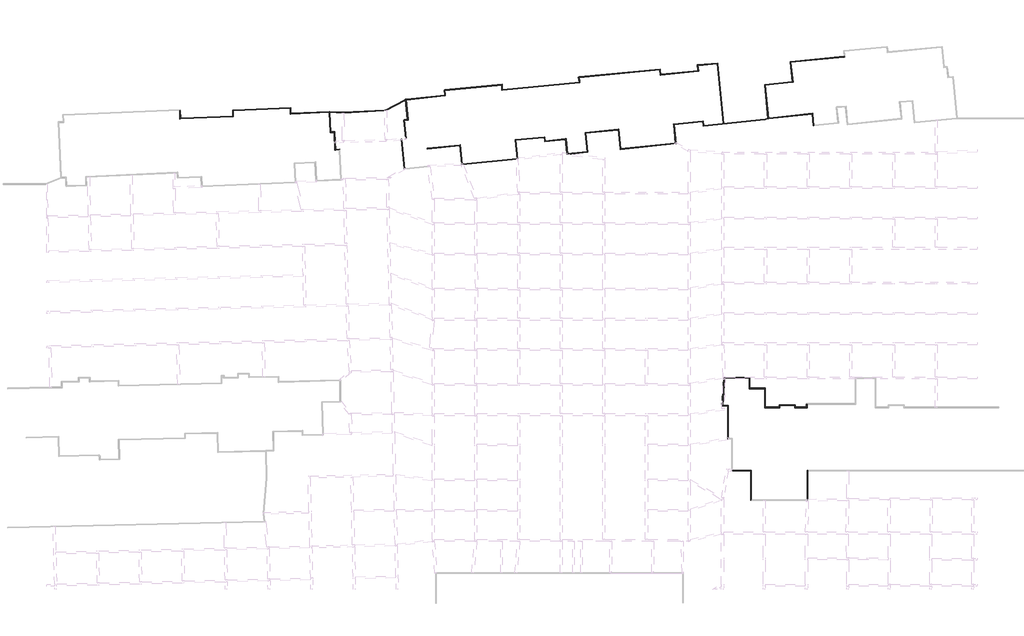
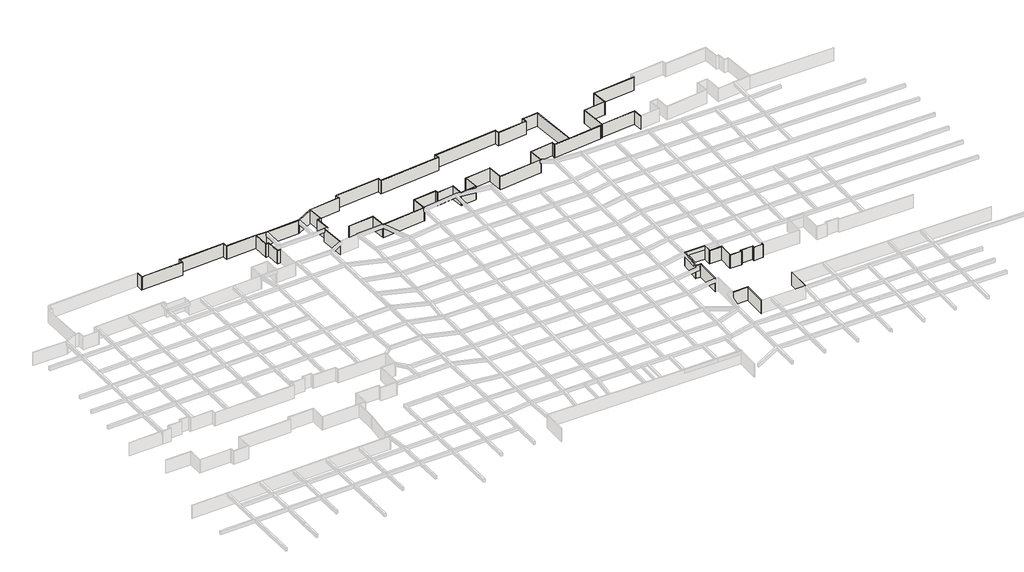
# One storey, part 6 of 20: 69 walls.
"""IFC4 building model written with IfcOpenShell, lengths in millimetres."""

from ifc_helpers import new_model, si_unit, origin, origin_with_axes, place, context, project, spatial, polyline, outline, extrude, faceted_brep, element, save

model = new_model("IFC4")

# Units and contexts
model_context = context("Model", 3, world=origin())
ifc_project = project(units=[si_unit("LENGTHUNIT", "METRE", prefix="MILLI")], contexts=[model_context])

# Site, building, storey
site = spatial("IfcSite", under=ifc_project)
building = spatial("IfcBuilding", under=site)
storey = spatial("IfcBuildingStorey", under=building, Name="户型图", Elevation=0.0)

# Walls
placement = place(None, origin())
element("IfcWall", 1, ObjectType="所有墙体", at=placement, inside=storey, context=model_context, shape_type="Brep", body=[
    faceted_brep([(131729.8124937, 210691.0787424, 0.0), (121574.8609355, 209733.4990588, 0.0), (121574.8609355, 209733.4990588, 3300.0), (131729.8124937, 210691.0787424, 3300.0), (131742.3566275, 210571.7292816, 0.0), (131742.3566275, 210571.7292816, 3300.0), (121706.8819283, 209625.4158865, 3300.0), (121587.4050693, 209614.1495981, 3300.0), (121587.4050693, 209614.1495981, 0.0), (121706.8819283, 209625.4158865, 0.0)], [[[0, 1, 2, 3]], [[4, 5, 6, 7, 8, 9]], [[1, 0, 4, 9, 8]], [[3, 2, 7, 6, 5]], [[0, 3, 5, 4]], [[2, 1, 8, 7]]]),
])
element("IfcWall", 2, ObjectType="所有墙体", at=placement, inside=storey, context=model_context, shape_type="Brep", body=[
    faceted_brep([(121587.4050693, 209614.1495981, 0.0), (121972.1365708, 205953.6738762, 0.0), (121984.6799864, 205834.3312487, 0.0), (121984.6799864, 205834.3312487, 3300.0), (121972.1365708, 205953.6738762, 3300.0), (121587.4050693, 209614.1495981, 3300.0), (121706.8819283, 209625.4158865, 0.0), (121706.8819283, 209625.4158865, 3300.0), (122104.0226138, 205846.8746643, 3300.0), (122104.0226138, 205846.8746643, 0.0)], [[[0, 1, 2, 3, 4, 5]], [[6, 7, 8, 9]], [[2, 1, 0, 6, 9]], [[5, 4, 3, 8, 7]], [[0, 5, 7, 6]], [[3, 2, 9, 8]]]),
])
element("IfcWall", 3, ObjectType="所有墙体", at=placement, inside=storey, context=model_context, shape_type="Brep", body=[
    faceted_brep([(121972.1365708, 205953.6738762, 0.0), (116800.5870466, 205410.1221183, 0.0), (116800.5870466, 205410.1221183, 3300.0), (121972.1365708, 205953.6738762, 3300.0), (121984.6799864, 205834.3312487, 0.0), (121984.6799864, 205834.3312487, 3300.0), (116931.2027957, 205303.1893932, 3300.0), (116811.853335, 205290.6452594, 3300.0), (116811.853335, 205290.6452594, 0.0), (116931.2027957, 205303.1893932, 0.0)], [[[0, 1, 2, 3]], [[4, 5, 6, 7, 8, 9]], [[1, 0, 4, 9, 8]], [[3, 2, 7, 6, 5]], [[0, 3, 5, 4]], [[2, 1, 8, 7]]]),
])
element("IfcWall", 4, ObjectType="所有墙体", at=placement, inside=storey, context=model_context, shape_type="Brep", body=[
    faceted_brep([(116811.853335, 205290.6452594, 0.0), (117393.2536778, 199125.0045105, 0.0), (117404.8959314, 199001.5406116, 0.0), (117404.8959314, 199001.5406116, 3300.0), (117393.2536778, 199125.0045105, 3300.0), (116811.853335, 205290.6452594, 3300.0), (116931.2027957, 205303.1893932, 0.0), (116931.2027957, 205303.1893932, 3300.0), (117521.4287148, 199043.9550761, 3300.0), (117521.4287148, 199043.9550761, 0.0)], [[[0, 1, 2, 3, 4, 5]], [[6, 7, 8, 9]], [[2, 1, 0, 6, 9]], [[5, 4, 3, 8, 7]], [[0, 5, 7, 6]], [[3, 2, 9, 8]]]),
])
element("IfcWall", 5, ObjectType="所有墙体", at=placement, inside=storey, context=model_context, shape_type="SweptSolid", body=[
    extrude(outline(polyline([(116894.9852677, 198943.6496406), (117393.2536778, 199125.0045105), (117404.8959314, 199001.5406116), (116922.1821154, 198825.8471509), (116894.9852677, 198943.6496406)])), origin_with_axes(), (0.0, 0.0, 1.0), 3300.0),
])
element("IfcWall", 6, ObjectType="所有墙体", at=placement, inside=storey, context=model_context, shape_type="Brep", body=[
    faceted_brep([(116894.9852677, 198943.6496406, 0.0), (109153.4306479, 198129.9794625, 0.0), (109034.0880204, 198117.4360469, 0.0), (105355.2231692, 197730.7717701, 0.0), (105235.8805418, 197718.2283545, 0.0), (105235.8805418, 197718.2283545, 3300.0), (105355.2231692, 197730.7717701, 3300.0), (109034.0880204, 198117.4360469, 3300.0), (109153.4306479, 198129.9794625, 3300.0), (116894.9852677, 198943.6496406, 3300.0), (116922.1821154, 198825.8471509, 0.0), (116922.1821154, 198825.8471509, 3300.0), (105248.4239574, 197598.885727, 3300.0), (105248.4239574, 197598.885727, 0.0)], [[[0, 1, 2, 3, 4, 5, 6, 7, 8, 9]], [[10, 11, 12, 13]], [[4, 3, 2, 1, 0, 10, 13]], [[9, 8, 7, 6, 5, 12, 11]], [[0, 9, 11, 10]], [[5, 4, 13, 12]]]),
])
element("IfcWall", 7, ObjectType="所有墙体", at=placement, inside=storey, context=model_context, shape_type="Brep", body=[
    faceted_brep([(105355.2231692, 197730.7717701, 0.0), (105266.7980678, 198572.0804116, 0.0), (105266.7980678, 198572.0804116, 3300.0), (105355.2231692, 197730.7717701, 3300.0), (105235.8805418, 197718.2283545, 0.0), (105235.8805418, 197718.2283545, 3300.0), (105159.998856, 198440.1943685, 3300.0), (105147.4554404, 198559.536996, 3300.0), (105147.4554404, 198559.536996, 0.0), (105159.998856, 198440.1943685, 0.0)], [[[0, 1, 2, 3]], [[4, 5, 6, 7, 8, 9]], [[1, 0, 4, 9, 8]], [[3, 2, 7, 6, 5]], [[0, 3, 5, 4]], [[2, 1, 8, 7]]]),
])
element("IfcWall", 8, ObjectType="所有墙体", at=placement, inside=storey, context=model_context, shape_type="Brep", body=[
    faceted_brep([(105147.4554404, 198559.536996, 0.0), (99683.6940432, 197985.2725327, 0.0), (99683.6940432, 197985.2725327, 3300.0), (105147.4554404, 198559.536996, 3300.0), (105159.998856, 198440.1943685, 0.0), (105159.998856, 198440.1943685, 3300.0), (99815.5800862, 197878.4733208, 3300.0), (99696.2374587, 197865.9299052, 3300.0), (99696.2374587, 197865.9299052, 0.0), (99815.5800862, 197878.4733208, 0.0)], [[[0, 1, 2, 3]], [[4, 5, 6, 7, 8, 9]], [[1, 0, 4, 9, 8]], [[3, 2, 7, 6, 5]], [[0, 3, 5, 4]], [[2, 1, 8, 7]]]),
])
element("IfcWall", 9, ObjectType="所有墙体", at=placement, inside=storey, context=model_context, shape_type="Brep", body=[
    faceted_brep([(99696.2374587, 197865.9299052, 0.0), (100056.1217007, 194441.8600656, 0.0), (100068.6651163, 194322.5174382, 0.0), (100068.6651163, 194322.5174382, 3300.0), (100056.1217007, 194441.8600656, 3300.0), (99696.2374587, 197865.9299052, 3300.0), (99815.5800862, 197878.4733208, 0.0), (99815.5800862, 197878.4733208, 3300.0), (100188.0077438, 194335.0608538, 3300.0), (100188.0077438, 194335.0608538, 0.0)], [[[0, 1, 2, 3, 4, 5]], [[6, 7, 8, 9]], [[2, 1, 0, 6, 9]], [[5, 4, 3, 8, 7]], [[0, 5, 7, 6]], [[3, 2, 9, 8]]]),
])
element("IfcWall", 10, ObjectType="所有墙体", at=placement, inside=storey, context=model_context, shape_type="Brep", body=[
    faceted_brep([(100056.1217007, 194441.8600656, 0.0), (89808.126809, 193364.7523995, 0.0), (89688.7841816, 193352.2089839, 0.0), (89688.7841816, 193352.2089839, 3300.0), (89808.126809, 193364.7523995, 3300.0), (100056.1217007, 194441.8600656, 3300.0), (100068.6651163, 194322.5174382, 0.0), (100068.6651163, 194322.5174382, 3300.0), (89701.3275972, 193232.8663565, 3300.0), (89701.3275972, 193232.8663565, 0.0)], [[[0, 1, 2, 3, 4, 5]], [[6, 7, 8, 9]], [[2, 1, 0, 6, 9]], [[5, 4, 3, 8, 7]], [[0, 5, 7, 6]], [[3, 2, 9, 8]]]),
])
element("IfcWall", 11, ObjectType="所有墙体", at=placement, inside=storey, context=model_context, shape_type="Brep", body=[
    faceted_brep([(89808.126809, 193364.7523995, 0.0), (89421.371495, 197044.4834124, 0.0), (89421.371495, 197044.4834124, 3300.0), (89808.126809, 193364.7523995, 3300.0), (89688.7841816, 193352.2089839, 0.0), (89688.7841816, 193352.2089839, 3300.0), (89314.5722831, 196912.5973693, 3300.0), (89302.0288675, 197031.9399968, 3300.0), (89302.0288675, 197031.9399968, 0.0), (89314.5722831, 196912.5973693, 0.0)], [[[0, 1, 2, 3]], [[4, 5, 6, 7, 8, 9]], [[1, 0, 4, 9, 8]], [[3, 2, 7, 6, 5]], [[0, 3, 5, 4]], [[2, 1, 8, 7]]]),
])
element("IfcWall", 12, ObjectType="所有墙体", at=placement, inside=storey, context=model_context, shape_type="Brep", body=[
    faceted_brep([(89302.0288675, 197031.9399968, 0.0), (83160.2882507, 196386.4170461, 0.0), (83160.2882507, 196386.4170461, 3300.0), (89302.0288675, 197031.9399968, 3300.0), (89314.5722831, 196912.5973693, 0.0), (89314.5722831, 196912.5973693, 3300.0), (83292.1742938, 196279.6178342, 3300.0), (83172.8316663, 196267.0744186, 3300.0), (83172.8316663, 196267.0744186, 0.0), (83292.1742938, 196279.6178342, 0.0)], [[[0, 1, 2, 3]], [[4, 5, 6, 7, 8, 9]], [[1, 0, 4, 9, 8]], [[3, 2, 7, 6, 5]], [[0, 3, 5, 4]], [[2, 1, 8, 7]]]),
])
element("IfcWall", 13, ObjectType="所有墙体", at=placement, inside=storey, context=model_context, shape_type="Brep", body=[
    faceted_brep([(83172.8316663, 196267.0744186, 0.0), (83535.1177075, 192820.1529861, 0.0), (83547.6611231, 192700.8103587, 0.0), (83547.6611231, 192700.8103587, 3300.0), (83535.1177075, 192820.1529861, 3300.0), (83172.8316663, 196267.0744186, 3300.0), (83292.1742938, 196279.6178342, 0.0), (83292.1742938, 196279.6178342, 3300.0), (83667.0037505, 192713.3537743, 3300.0), (83667.0037505, 192713.3537743, 0.0)], [[[0, 1, 2, 3, 4, 5]], [[6, 7, 8, 9]], [[2, 1, 0, 6, 9]], [[5, 4, 3, 8, 7]], [[0, 5, 7, 6]], [[3, 2, 9, 8]]]),
])
element("IfcWall", 14, ObjectType="所有墙体", at=placement, inside=storey, context=model_context, shape_type="Brep", body=[
    faceted_brep([(83535.1177075, 192820.1529861, 0.0), (79847.9790856, 192432.6191009, 0.0), (79728.6364581, 192420.0756853, 0.0), (79728.6364581, 192420.0756853, 3300.0), (79847.9790856, 192432.6191009, 3300.0), (80284.9846417, 192478.5502357, 3300.0), (83535.1177075, 192820.1529861, 3300.0), (83547.6611231, 192700.8103587, 0.0), (83547.6611231, 192700.8103587, 3300.0), (80814.4577688, 192413.5391103, 3300.0), (79741.1798737, 192300.7330579, 3300.0), (79741.1798737, 192300.7330579, 2500.0), (79741.1798737, 192300.7330579, 0.0)], [[[0, 1, 2, 3, 4, 5, 6]], [[7, 8, 9, 10, 11, 12]], [[2, 1, 0, 7, 12]], [[6, 5, 4, 3, 10, 9, 8]], [[0, 6, 8, 7]], [[3, 2, 12, 11, 10]]]),
])
element("IfcWall", 15, ObjectType="所有墙体", at=placement, inside=storey, context=model_context, shape_type="Brep", body=[
    faceted_brep([(79847.9790856, 192432.6191009, 0.0), (79552.5957881, 195243.0034464, 0.0), (79552.5957881, 195243.0034464, 3300.0), (79837.3750476, 192533.5097832, 3300.0), (79847.9790856, 192432.6191009, 3300.0), (79847.9790856, 192432.6191009, 2500.0), (79728.6364581, 192420.0756853, 0.0), (79728.6364581, 192420.0756853, 3300.0), (79715.1365445, 192548.5187841, 3300.0), (79445.7965763, 195111.1174033, 3300.0), (79433.2531607, 195230.4600308, 3300.0), (79433.2531607, 195230.4600308, 0.0), (79445.7965763, 195111.1174033, 0.0)], [[[0, 1, 2, 3, 4, 5]], [[6, 7, 8, 9, 10, 11, 12]], [[1, 0, 6, 12, 11]], [[4, 3, 2, 10, 9, 8, 7]], [[0, 5, 4, 7, 6]], [[2, 1, 11, 10]]]),
])
element("IfcWall", 16, ObjectType="所有墙体", at=placement, inside=storey, context=model_context, shape_type="Brep", body=[
    faceted_brep([(79433.2531607, 195230.4600308, 0.0), (75644.1175717, 194832.2058324, 0.0), (75524.7749443, 194819.6624168, 0.0), (75524.7749443, 194819.6624168, 3300.0), (75644.1175717, 194832.2058324, 3300.0), (79433.2531607, 195230.4600308, 3300.0), (79445.7965763, 195111.1174033, 0.0), (79445.7965763, 195111.1174033, 3300.0), (75537.3183598, 194700.3197894, 3300.0), (75537.3183598, 194700.3197894, 0.0)], [[[0, 1, 2, 3, 4, 5]], [[6, 7, 8, 9]], [[2, 1, 0, 6, 9]], [[5, 4, 3, 8, 7]], [[0, 5, 7, 6]], [[3, 2, 9, 8]]]),
])
element("IfcWall", 17, ObjectType="所有墙体", at=placement, inside=storey, context=model_context, shape_type="Brep", body=[
    faceted_brep([(75644.1175717, 194832.2058324, 0.0), (75564.7799301, 195587.0530699, 0.0), (75564.7799301, 195587.0530699, 3300.0), (75644.1175717, 194832.2058324, 3300.0), (75524.7749443, 194819.6624168, 0.0), (75524.7749443, 194819.6624168, 3300.0), (75457.7636828, 195457.2319809, 3300.0), (75445.2183565, 195576.5927876, 3300.0), (75445.2183565, 195576.5927876, 0.0), (75457.7636828, 195457.2319809, 0.0)], [[[0, 1, 2, 3]], [[4, 5, 6, 7, 8, 9]], [[1, 0, 4, 9, 8]], [[3, 2, 7, 6, 5]], [[0, 3, 5, 4]], [[2, 1, 8, 7]]]),
])
element("IfcWall", 18, ObjectType="所有墙体", at=placement, inside=storey, context=model_context, shape_type="Brep", body=[
    faceted_brep([(75445.2183565, 195576.5927876, 0.0), (69986.0714109, 195098.9793173, 0.0), (69986.0714109, 195098.9793173, 3300.0), (75445.2183565, 195576.5927876, 3300.0), (75457.7636828, 195457.2319809, 0.0), (75457.7636828, 195457.2319809, 3300.0), (70118.1783108, 194990.0787929, 3300.0), (69998.6167372, 194979.6185106, 3300.0), (69998.6167372, 194979.6185106, 0.0), (70118.1783108, 194990.0787929, 0.0)], [[[0, 1, 2, 3]], [[4, 5, 6, 7, 8, 9]], [[1, 0, 4, 9, 8]], [[3, 2, 7, 6, 5]], [[0, 3, 5, 4]], [[2, 1, 8, 7]]]),
])
element("IfcWall", 19, ObjectType="所有墙体", at=placement, inside=storey, context=model_context, shape_type="Brep", body=[
    faceted_brep([(69998.6167372, 194979.6185106, 0.0), (70362.4316658, 191518.1506866, 0.0), (70374.9755195, 191398.8038903, 0.0), (70374.9755195, 191398.8038903, 3300.0), (70362.4316658, 191518.1506866, 3300.0), (69998.6167372, 194979.6185106, 3300.0), (70118.1783108, 194990.0787929, 0.0), (70118.1783108, 194990.0787929, 3300.0), (70494.4229915, 191410.349777, 3300.0), (70494.4229915, 191410.349777, 0.0)], [[[0, 1, 2, 3, 4, 5]], [[6, 7, 8, 9]], [[2, 1, 0, 6, 9]], [[5, 4, 3, 8, 7]], [[0, 5, 7, 6]], [[3, 2, 9, 8]]]),
])
element("IfcWall", 20, ObjectType="所有墙体", at=placement, inside=storey, context=model_context, shape_type="Brep", body=[
    faceted_brep([(70362.4316658, 191518.1506866, 0.0), (60092.4518091, 190525.4463415, 0.0), (59973.0043371, 190513.9004548, 0.0), (59973.0043371, 190513.9004548, 3300.0), (60092.4518091, 190525.4463415, 3300.0), (70362.4316658, 191518.1506866, 3300.0), (70374.9755195, 191398.8038903, 0.0), (70374.9755195, 191398.8038903, 3300.0), (59985.5481909, 190394.5536585, 3300.0), (59985.5481909, 190394.5536585, 0.0)], [[[0, 1, 2, 3, 4, 5]], [[6, 7, 8, 9]], [[2, 1, 0, 6, 9]], [[5, 4, 3, 8, 7]], [[0, 5, 7, 6]], [[3, 2, 9, 8]]]),
])
element("IfcWall", 21, ObjectType="所有墙体", at=placement, inside=storey, context=model_context, shape_type="Brep", body=[
    faceted_brep([(60092.4518091, 190525.4463415, 0.0), (59716.0971382, 194106.2218448, 0.0), (59716.0971382, 194106.2218448, 3300.0), (60092.4518091, 190525.4463415, 3300.0), (59973.0043371, 190513.9004548, 0.0), (59973.0043371, 190513.9004548, 3300.0), (59609.2979263, 193974.3358018, 3300.0), (59596.7545107, 194093.6784293, 3300.0), (59596.7545107, 194093.6784293, 0.0), (59609.2979263, 193974.3358018, 0.0)], [[[0, 1, 2, 3]], [[4, 5, 6, 7, 8, 9]], [[1, 0, 4, 9, 8]], [[3, 2, 7, 6, 5]], [[0, 3, 5, 4]], [[2, 1, 8, 7]]]),
])
element("IfcWall", 22, ObjectType="所有墙体", at=placement, inside=storey, context=model_context, shape_type="SweptSolid", body=[
    extrude(outline(polyline([(53516.2635964, 193454.5930817), (59596.7545107, 194093.6784293), (59609.2979263, 193974.3358018), (53528.8070119, 193335.2504542), (53516.2635964, 193454.5930817)])), origin_with_axes(), (0.0, 0.0, 1.0), 3300.0),
])
element("IfcWall", 23, ObjectType="所有墙体", at=placement, inside=storey, context=model_context, shape_type="Brep", body=[
    faceted_brep([(48667.2783502, 195165.2272583, 0.0), (49211.8887729, 189530.9836906, 0.0), (49211.8887729, 189530.9836906, 3300.0), (48684.0697224, 194991.5128437, 3300.0), (48667.2783502, 195165.2272583, 3300.0), (48667.2783502, 195165.2272583, 2500.0), (48786.7216498, 195176.7727417, 0.0), (48786.7216498, 195176.7727417, 2500.0), (48786.7216498, 195176.7727417, 3300.0), (48803.4165187, 195004.0566974, 3300.0), (49319.6896824, 189662.9750163, 3300.0), (49331.2355692, 189543.5275444, 3300.0), (49331.2355692, 189543.5275444, 0.0), (49319.6896824, 189662.9750163, 0.0)], [[[0, 1, 2, 3, 4, 5]], [[6, 7, 8, 9, 10, 11, 12, 13]], [[1, 0, 6, 13, 12]], [[4, 3, 2, 11, 10, 9, 8]], [[0, 5, 4, 8, 7, 6]], [[2, 1, 12, 11]]]),
])
element("IfcWall", 24, ObjectType="所有墙体", at=placement, inside=storey, context=model_context, shape_type="Brep", body=[
    faceted_brep([(49582.7742245, 195254.2236424, 0.0), (49223.1963109, 198675.3789625, 0.0), (49210.6528953, 198794.7215899, 0.0), (49210.6528953, 198794.7215899, 3300.0), (49223.1963109, 198675.3789625, 3300.0), (49582.7742245, 195254.2236424, 3300.0), (49463.4315971, 195241.6802268, 0.0), (49463.4315971, 195241.6802268, 3300.0), (49091.3102679, 198782.1781744, 3300.0), (49091.3102679, 198782.1781744, 0.0)], [[[0, 1, 2, 3, 4, 5]], [[6, 7, 8, 9]], [[2, 1, 0, 6, 9]], [[5, 4, 3, 8, 7]], [[0, 5, 7, 6]], [[3, 2, 9, 8]]]),
])
element("IfcWall", 25, ObjectType="所有墙体", at=placement, inside=storey, context=model_context, shape_type="Brep", body=[
    faceted_brep([(49223.1963109, 198675.3789625, 0.0), (49941.1246624, 198750.8362729, 0.0), (49941.1246624, 198750.8362729, 3300.0), (49223.1963109, 198675.3789625, 3300.0), (49210.6528953, 198794.7215899, 0.0), (49210.6528953, 198794.7215899, 3300.0), (49810.2319794, 198857.7398911, 3300.0), (49929.5787757, 198870.2837448, 3300.0), (49929.5787757, 198870.2837448, 0.0), (49810.2319794, 198857.7398911, 0.0)], [[[0, 1, 2, 3]], [[4, 5, 6, 7, 8, 9]], [[1, 0, 4, 9, 8]], [[3, 2, 7, 6, 5]], [[0, 3, 5, 4]], [[2, 1, 8, 7]]]),
])
element("IfcWall", 26, ObjectType="所有墙体", at=placement, inside=storey, context=model_context, shape_type="Brep", body=[
    faceted_brep([(49929.5787757, 198870.2837448, 0.0), (49575.5176865, 202533.2074259, 0.0), (49563.9717998, 202652.6548978, 0.0), (49563.9717998, 202652.6548978, 3300.0), (49575.5176865, 202533.2074259, 3300.0), (49929.5787757, 198870.2837448, 3300.0), (49810.2319794, 198857.7398911, 0.0), (49810.2319794, 198857.7398911, 3300.0), (49458.9857705, 202491.5423501, 3300.0), (49446.4909346, 202620.8071341, 3300.0), (49444.6250035, 202640.1110441, 3300.0), (49444.6250035, 202640.1110441, 0.0), (49446.4909346, 202620.8071341, 0.0), (49458.9857705, 202491.5423501, 0.0)], [[[0, 1, 2, 3, 4, 5]], [[6, 7, 8, 9, 10, 11, 12, 13]], [[2, 1, 0, 6, 13, 12, 11]], [[5, 4, 3, 10, 9, 8, 7]], [[0, 5, 7, 6]], [[3, 2, 11, 10]]]),
])
element("IfcWall", 27, ObjectType="所有墙体", at=placement, inside=storey, context=model_context, shape_type="Brep", body=[
    faceted_brep([(49575.5176865, 202533.2074259, 0.0), (56935.4763922, 203306.7702572, 0.0), (56935.4763922, 203306.7702572, 3300.0), (49575.5176865, 202533.2074259, 3300.0), (49563.9717998, 202652.6548978, 0.0), (49563.9717998, 202652.6548978, 3300.0), (56803.5903492, 203413.5694691, 3300.0), (56922.9329766, 203426.1128847, 3300.0), (56922.9329766, 203426.1128847, 0.0), (56803.5903492, 203413.5694691, 0.0)], [[[0, 1, 2, 3]], [[4, 5, 6, 7, 8, 9]], [[1, 0, 4, 9, 8]], [[3, 2, 7, 6, 5]], [[0, 3, 5, 4]], [[2, 1, 8, 7]]]),
])
element("IfcWall", 28, ObjectType="所有墙体", at=placement, inside=storey, context=model_context, shape_type="Brep", body=[
    faceted_brep([(56922.9329766, 203426.1128847, 0.0), (56831.5181439, 204295.8669196, 0.0), (56818.9742902, 204415.2137159, 0.0), (56818.9742902, 204415.2137159, 3300.0), (56831.5181439, 204295.8669196, 3300.0), (56922.9329766, 203426.1128847, 3300.0), (56803.5903492, 203413.5694691, 0.0), (56803.5903492, 203413.5694691, 3300.0), (56699.5268182, 204403.6678292, 3300.0), (56699.5268182, 204403.6678292, 0.0)], [[[0, 1, 2, 3, 4, 5]], [[6, 7, 8, 9]], [[2, 1, 0, 6, 9]], [[5, 4, 3, 8, 7]], [[0, 5, 7, 6]], [[3, 2, 9, 8]]]),
])
element("IfcWall", 29, ObjectType="所有墙体", at=placement, inside=storey, context=model_context, shape_type="Brep", body=[
    faceted_brep([(56831.5181439, 204295.8669196, 0.0), (67455.4194423, 205322.7815901, 0.0), (67575.4194423, 205334.3808846, 0.0), (67575.4194423, 205334.3808846, 3300.0), (67455.4194423, 205322.7815901, 3300.0), (56831.5181439, 204295.8669196, 3300.0), (56818.9742902, 204415.2137159, 0.0), (56818.9742902, 204415.2137159, 3300.0), (67575.4194423, 205454.9401797, 3300.0), (67575.4194423, 205454.9401797, 0.0)], [[[0, 1, 2, 3, 4, 5]], [[6, 7, 8, 9]], [[2, 1, 0, 6, 9]], [[5, 4, 3, 8, 7]], [[0, 5, 7, 6]], [[3, 2, 9, 8]]]),
])
element("IfcWall", 30, ObjectType="所有墙体", at=placement, inside=storey, context=model_context, shape_type="Brep", body=[
    faceted_brep([(67455.4194423, 205322.7815901, 0.0), (67455.4194423, 204322.7815901, 0.0), (67455.4194423, 204322.7815901, 3300.0), (67455.4194423, 205322.7815901, 3300.0), (67575.4194423, 205334.3808846, 0.0), (67575.4194423, 205334.3808846, 3300.0), (67575.4194423, 204454.9401797, 3300.0), (67575.4194423, 204334.3808846, 3300.0), (67575.4194423, 204334.3808846, 0.0), (67575.4194423, 204454.9401797, 0.0)], [[[0, 1, 2, 3]], [[4, 5, 6, 7, 8, 9]], [[1, 0, 4, 9, 8]], [[3, 2, 7, 6, 5]], [[0, 3, 5, 4]], [[2, 1, 8, 7]]]),
])
element("IfcWall", 31, ObjectType="所有墙体", at=placement, inside=storey, context=model_context, shape_type="Brep", body=[
    faceted_brep([(67575.4194423, 204334.3808846, 0.0), (82113.181948, 205739.6124633, 0.0), (82113.181948, 205739.6124633, 3300.0), (67575.4194423, 204334.3808846, 3300.0), (67575.4194423, 204454.9401797, 0.0), (67575.4194423, 204454.9401797, 3300.0), (81982.193165, 205847.5102794, 3300.0), (82101.6364646, 205859.0557628, 3300.0), (82101.6364646, 205859.0557628, 0.0), (81982.193165, 205847.5102794, 0.0)], [[[0, 1, 2, 3]], [[4, 5, 6, 7, 8, 9]], [[1, 0, 4, 9, 8]], [[3, 2, 7, 6, 5]], [[0, 3, 5, 4]], [[2, 1, 8, 7]]]),
])
element("IfcWall", 32, ObjectType="所有墙体", at=placement, inside=storey, context=model_context, shape_type="Brep", body=[
    faceted_brep([(81886.4271484, 206838.2534608, 0.0), (81982.193165, 205847.5102794, 0.0), (81982.193165, 205847.5102794, 3300.0), (81886.4271484, 206838.2534608, 3300.0), (82005.870448, 206849.7989442, 0.0), (82005.870448, 206849.7989442, 3300.0), (82017.4159314, 206730.3556446, 3300.0), (82101.6364646, 205859.0557628, 3300.0), (82101.6364646, 205859.0557628, 0.0), (82017.4159314, 206730.3556446, 0.0)], [[[0, 1, 2, 3]], [[4, 5, 6, 7, 8, 9]], [[1, 0, 4, 9, 8]], [[3, 2, 7, 6, 5]], [[2, 1, 8, 7]], [[0, 3, 5, 4]]]),
])
element("IfcWall", 33, ObjectType="所有墙体", at=placement, inside=storey, context=model_context, shape_type="Brep", body=[
    faceted_brep([(82017.4159314, 206730.3556446, 0.0), (97124.0566493, 208190.5754395, 0.0), (97243.4999488, 208202.120923, 0.0), (97243.4999488, 208202.120923, 3300.0), (97124.0566493, 208190.5754395, 3300.0), (82017.4159314, 206730.3556446, 3300.0), (82005.870448, 206849.7989442, 0.0), (82005.870448, 206849.7989442, 3300.0), (97231.9544654, 208321.5642225, 3300.0), (97231.9544654, 208321.5642225, 0.0)], [[[0, 1, 2, 3, 4, 5]], [[6, 7, 8, 9]], [[2, 1, 0, 6, 9]], [[5, 4, 3, 8, 7]], [[0, 5, 7, 6]], [[3, 2, 9, 8]]]),
])
element("IfcWall", 34, ObjectType="所有墙体", at=placement, inside=storey, context=model_context, shape_type="Brep", body=[
    faceted_brep([(97124.0566493, 208190.5754395, 0.0), (97219.1952312, 207206.3233554, 0.0), (97219.1952312, 207206.3233554, 3300.0), (97124.0566493, 208190.5754395, 3300.0), (97243.4999488, 208202.120923, 0.0), (97243.4999488, 208202.120923, 3300.0), (97327.0930474, 207337.3121384, 3300.0), (97338.6385308, 207217.8688388, 3300.0), (97338.6385308, 207217.8688388, 0.0), (97327.0930474, 207337.3121384, 0.0)], [[[0, 1, 2, 3]], [[4, 5, 6, 7, 8, 9]], [[1, 0, 4, 9, 8]], [[3, 2, 7, 6, 5]], [[0, 3, 5, 4]], [[2, 1, 8, 7]]]),
])
element("IfcWall", 35, ObjectType="所有墙体", at=placement, inside=storey, context=model_context, shape_type="Brep", body=[
    faceted_brep([(97338.6385308, 207217.8688388, 0.0), (104406.2016933, 207901.0250629, 0.0), (104406.2016933, 207901.0250629, 3300.0), (97338.6385308, 207217.8688388, 3300.0), (97327.0930474, 207337.3121384, 0.0), (97327.0930474, 207337.3121384, 3300.0), (104274.2103676, 208008.8259724, 3300.0), (104393.6578396, 208020.3718592, 3300.0), (104393.6578396, 208020.3718592, 0.0), (104274.2103676, 208008.8259724, 0.0)], [[[0, 1, 2, 3]], [[4, 5, 6, 7, 8, 9]], [[1, 0, 4, 9, 8]], [[3, 2, 7, 6, 5]], [[0, 3, 5, 4]], [[2, 1, 8, 7]]]),
])
element("IfcWall", 36, ObjectType="所有墙体", at=placement, inside=storey, context=model_context, shape_type="Brep", body=[
    faceted_brep([(104393.6578396, 208020.3718592, 0.0), (104291.2203837, 208994.9991478, 0.0), (104278.67653, 209114.3459441, 0.0), (104278.67653, 209114.3459441, 3300.0), (104291.2203837, 208994.9991478, 3300.0), (104393.6578396, 208020.3718592, 3300.0), (104274.2103676, 208008.8259724, 0.0), (104274.2103676, 208008.8259724, 3300.0), (104159.229058, 209102.8000573, 3300.0), (104159.229058, 209102.8000573, 0.0)], [[[0, 1, 2, 3, 4, 5]], [[6, 7, 8, 9]], [[2, 1, 0, 6, 9]], [[5, 4, 3, 8, 7]], [[0, 5, 7, 6]], [[3, 2, 9, 8]]]),
])
element("IfcWall", 37, ObjectType="所有墙体", at=placement, inside=storey, context=model_context, shape_type="Brep", body=[
    faceted_brep([(104291.2203837, 208994.9991478, 0.0), (107854.6079818, 209339.4390007, 0.0), (107974.0554538, 209350.9848875, 0.0), (107974.0554538, 209350.9848875, 3300.0), (107854.6079818, 209339.4390007, 3300.0), (104291.2203837, 208994.9991478, 3300.0), (104278.67653, 209114.3459441, 0.0), (104278.67653, 209114.3459441, 3300.0), (107961.5116, 209470.3316838, 3300.0), (107961.5116, 209470.3316838, 0.0)], [[[0, 1, 2, 3, 4, 5]], [[6, 7, 8, 9]], [[2, 1, 0, 6, 9]], [[5, 4, 3, 8, 7]], [[0, 5, 7, 6]], [[3, 2, 9, 8]]]),
])
element("IfcWall", 38, ObjectType="所有墙体", at=placement, inside=storey, context=model_context, shape_type="SweptSolid", body=[
    extrude(outline(polyline([(109034.0880204, 198117.4360469), (107854.6079818, 209339.4390007), (107974.0554538, 209350.9848875), (109153.4306479, 198129.9794625), (109034.0880204, 198117.4360469)])), origin_with_axes(), (0.0, 0.0, 1.0), 3300.0),
])
element("IfcWall", 39, ObjectType="所有墙体", at=placement, inside=storey, context=model_context, shape_type="Brep", body=[
    faceted_brep([(49446.4909346, 202620.8071341, 0.0), (45696.9730881, 200627.153131, 0.0), (45446.265249, 200493.8494083, 0.0), (45446.265249, 200493.8494083, 3300.0), (45696.9730881, 200627.153131, 3300.0), (49446.4909346, 202620.8071341, 3300.0), (49458.9857705, 202491.5423501, 0.0), (49458.9857705, 202491.5423501, 3300.0), (45729.8203033, 200508.709899, 3300.0), (45729.8203033, 200508.709899, 0.0)], [[[0, 1, 2, 3, 4, 5]], [[6, 7, 8, 9]], [[2, 1, 0, 6, 9]], [[5, 4, 3, 8, 7]], [[0, 5, 7, 6]], [[3, 2, 9, 8]]]),
])
element("IfcWall", 40, ObjectType="所有墙体", at=placement, inside=storey, context=model_context, shape_type="SweptSolid", body=[
    extrude(outline(polyline([(37724.3604177, 200209.3262058), (45696.9730881, 200627.153131), (45446.265249, 200493.8494083), (37724.3604177, 200089.1615243), (37724.3604177, 200209.3262058)])), origin_with_axes(), (0.0, 0.0, 1.0), 3300.0),
])
element("IfcWall", 41, ObjectType="所有墙体", at=placement, inside=storey, context=model_context, shape_type="Brep", body=[
    faceted_brep([(37724.3604177, 200209.3262058, 0.0), (35164.3813106, 200343.4890258, 0.0), (35164.3813106, 200343.4890258, 3300.0), (37724.3604177, 200209.3262058, 3300.0), (37724.3604177, 200089.1615243, 0.0), (37724.3604177, 200089.1615243, 3300.0), (35291.1918509, 200216.6784855, 3300.0), (35170.6962191, 200222.993394, 3300.0), (35170.6962191, 200222.993394, 0.0), (35291.1918509, 200216.6784855, 0.0)], [[[0, 1, 2, 3]], [[4, 5, 6, 7, 8, 9]], [[1, 0, 4, 9, 8]], [[3, 2, 7, 6, 5]], [[0, 3, 5, 4]], [[2, 1, 8, 7]]]),
])
element("IfcWall", 42, ObjectType="所有墙体", at=placement, inside=storey, context=model_context, shape_type="Brep", body=[
    faceted_brep([(35170.6962191, 200222.993394, 0.0), (35369.7253405, 196425.2915236, 0.0), (35369.7253405, 196425.2915236, 3300.0), (35170.6962191, 200222.993394, 3300.0), (35291.1918509, 200216.6784855, 0.0), (35291.1918509, 200216.6784855, 3300.0), (35483.6010885, 196545.2915236, 3300.0), (35489.890022, 196425.2915236, 3300.0), (35489.890022, 196425.2915236, 0.0), (35483.6010885, 196545.2915236, 0.0)], [[[0, 1, 2, 3]], [[4, 5, 6, 7, 8, 9]], [[1, 0, 4, 9, 8]], [[3, 2, 7, 6, 5]], [[0, 3, 5, 4]], [[2, 1, 8, 7]]]),
])
element("IfcWall", 43, ObjectType="所有墙体", at=placement, inside=storey, context=model_context, shape_type="Brep", body=[
    faceted_brep([(35489.890022, 196425.2915236, 0.0), (36069.7253405, 196425.2915236, 0.0), (36189.890022, 196425.2915236, 0.0), (36189.890022, 196425.2915236, 3300.0), (36069.7253405, 196425.2915236, 3300.0), (35489.890022, 196425.2915236, 3300.0), (35483.6010885, 196545.2915236, 0.0), (35483.6010885, 196545.2915236, 3300.0), (36183.6010885, 196545.2915236, 3300.0), (36183.6010885, 196545.2915236, 0.0)], [[[0, 1, 2, 3, 4, 5]], [[6, 7, 8, 9]], [[2, 1, 0, 6, 9]], [[5, 4, 3, 8, 7]], [[0, 5, 7, 6]], [[3, 2, 9, 8]]]),
])
element("IfcWall", 44, ObjectType="所有墙体", at=placement, inside=storey, context=model_context, shape_type="Brep", body=[
    faceted_brep([(36069.7253405, 196425.2915236, 0.0), (36242.5942554, 193126.7561294, 0.0), (36242.5942554, 193126.7561294, 3300.0), (36069.7253405, 196425.2915236, 3300.0), (36189.890022, 196425.2915236, 0.0), (36189.890022, 196425.2915236, 3300.0), (36356.1494848, 193252.8719884, 3300.0), (36362.4297996, 193133.0364442, 3300.0), (36362.4297996, 193133.0364442, 0.0), (36356.1494848, 193252.8719884, 0.0)], [[[0, 1, 2, 3]], [[4, 5, 6, 7, 8, 9]], [[1, 0, 4, 9, 8]], [[3, 2, 7, 6, 5]], [[0, 3, 5, 4]], [[2, 1, 8, 7]]]),
])
element("IfcWall", 45, ObjectType="所有墙体", at=placement, inside=storey, context=model_context, shape_type="Brep", body=[
    faceted_brep([(36362.4297996, 193133.0364442, 0.0), (37019.504808, 193167.4722862, 0.0), (37139.3403522, 193173.752601, 0.0), (37139.3403522, 193173.752601, 3300.0), (37019.504808, 193167.4722862, 3300.0), (36362.4297996, 193133.0364442, 3300.0), (36356.1494848, 193252.8719884, 0.0), (36356.1494848, 193252.8719884, 3300.0), (37133.0600374, 193293.5881451, 3300.0), (37133.0600374, 193293.5881451, 0.0)], [[[0, 1, 2, 3, 4, 5]], [[6, 7, 8, 9]], [[2, 1, 0, 6, 9]], [[5, 4, 3, 8, 7]], [[0, 5, 7, 6]], [[3, 2, 9, 8]]]),
])
element("IfcWall", 46, ObjectType="所有墙体", at=placement, inside=storey, context=model_context, shape_type="Brep", body=[
    faceted_brep([(7101.7994998, 200617.8498929, 0.0), (7175.1900793, 198971.4081549, 0.0), (7175.1900793, 198971.4081549, 3300.0), (7101.7994998, 200617.8498929, 3300.0), (7221.6804599, 200623.1936187, 0.0), (7221.6804599, 200623.1936187, 3300.0), (7289.7273137, 199096.6328407, 3300.0), (7295.0710394, 198976.7518806, 3300.0), (7295.0710394, 198976.7518806, 0.0), (7289.7273137, 199096.6328407, 0.0)], [[[0, 1, 2, 3]], [[4, 5, 6, 7, 8, 9]], [[1, 0, 4, 9, 8]], [[3, 2, 7, 6, 5]], [[0, 3, 5, 4]], [[2, 1, 8, 7]]]),
])
element("IfcWall", 47, ObjectType="所有墙体", at=placement, inside=storey, context=model_context, shape_type="Brep", body=[
    faceted_brep([(7295.0710394, 198976.7518806, 0.0), (17183.0494545, 199417.5111552, 0.0), (17183.0494545, 199417.5111552, 3300.0), (7295.0710394, 198976.7518806, 3300.0), (7289.7273137, 199096.6328407, 0.0), (7289.7273137, 199096.6328407, 3300.0), (17063.0494545, 199532.2812813, 3300.0), (17183.0494545, 199537.6303133, 3300.0), (17183.0494545, 199537.6303133, 0.0), (17063.0494545, 199532.2812813, 0.0)], [[[0, 1, 2, 3]], [[4, 5, 6, 7, 8, 9]], [[1, 0, 4, 9, 8]], [[3, 2, 7, 6, 5]], [[0, 3, 5, 4]], [[2, 1, 8, 7]]]),
])
element("IfcWall", 48, ObjectType="所有墙体", at=placement, inside=storey, context=model_context, shape_type="Brep", body=[
    faceted_brep([(17183.0494545, 199537.6303133, 0.0), (17183.0494545, 200517.5111552, 0.0), (17183.0494545, 200637.6303133, 0.0), (17183.0494545, 200637.6303133, 3300.0), (17183.0494545, 200517.5111552, 3300.0), (17183.0494545, 199537.6303133, 3300.0), (17063.0494545, 199532.2812813, 0.0), (17063.0494545, 199532.2812813, 3300.0), (17063.0494545, 200632.2812813, 3300.0), (17063.0494545, 200632.2812813, 0.0)], [[[0, 1, 2, 3, 4, 5]], [[6, 7, 8, 9]], [[2, 1, 0, 6, 9]], [[5, 4, 3, 8, 7]], [[0, 5, 7, 6]], [[3, 2, 9, 8]]]),
])
element("IfcWall", 49, ObjectType="所有墙体", at=placement, inside=storey, context=model_context, shape_type="Brep", body=[
    faceted_brep([(17183.0494545, 200517.5111552, 0.0), (27852.3358636, 200993.0974419, 0.0), (27972.3358636, 200998.4464739, 0.0), (27972.3358636, 200998.4464739, 3300.0), (27852.3358636, 200993.0974419, 3300.0), (17183.0494545, 200517.5111552, 3300.0), (17183.0494545, 200637.6303133, 0.0), (17183.0494545, 200637.6303133, 3300.0), (27972.3358636, 201118.565632, 3300.0), (27972.3358636, 201118.565632, 0.0)], [[[0, 1, 2, 3, 4, 5]], [[6, 7, 8, 9]], [[2, 1, 0, 6, 9]], [[5, 4, 3, 8, 7]], [[0, 5, 7, 6]], [[3, 2, 9, 8]]]),
])
element("IfcWall", 50, ObjectType="所有墙体", at=placement, inside=storey, context=model_context, shape_type="Brep", body=[
    faceted_brep([(27852.3358636, 200993.0974419, 0.0), (27852.3358636, 199893.0974419, 0.0), (27852.3358636, 199893.0974419, 3300.0), (27852.3358636, 200993.0974419, 3300.0), (27972.3358636, 200998.4464739, 0.0), (27972.3358636, 200998.4464739, 3300.0), (27972.3358636, 200018.565632, 3300.0), (27972.3358636, 199898.4464739, 3300.0), (27972.3358636, 199898.4464739, 0.0), (27972.3358636, 200018.565632, 0.0)], [[[0, 1, 2, 3]], [[4, 5, 6, 7, 8, 9]], [[1, 0, 4, 9, 8]], [[3, 2, 7, 6, 5]], [[0, 3, 5, 4]], [[2, 1, 8, 7]]]),
])
element("IfcWall", 51, ObjectType="所有墙体", at=placement, inside=storey, context=model_context, shape_type="SweptSolid", body=[
    extrude(outline(polyline([(35230.36245, 200221.9749444), (27972.3358636, 199898.4464739), (27972.3358636, 200018.565632), (35225.0187242, 200341.8559045), (35230.36245, 200221.9749444)])), origin_with_axes(), (0.0, 0.0, 1.0), 3300.0),
])
element("IfcWall", 52, ObjectType="所有墙体", at=placement, inside=storey, context=model_context, shape_type="Brep", body=[
    faceted_brep([(117470.9396202, 199025.5785485, 0.0), (125657.8313417, 199886.0555421, 0.0), (125777.1808024, 199898.5996759, 0.0), (125777.1808024, 199898.5996759, 3300.0), (125657.8313417, 199886.0555421, 3300.0), (117470.9396202, 199025.5785485, 3300.0), (117511.3827825, 199150.4902897, 0.0), (117511.3827825, 199150.4902897, 3300.0), (125765.9145141, 200018.0765348, 3300.0), (125765.9145141, 200018.0765348, 0.0), (117521.4287148, 199043.9550761, 0.0), (117521.4287148, 199043.9550761, 3300.0)], [[[0, 1, 2, 3, 4, 5]], [[6, 7, 8, 9]], [[2, 1, 0, 10, 6, 9]], [[5, 4, 3, 8, 7, 11]], [[3, 2, 9, 8]], [[0, 5, 11, 10]], [[11, 7, 6, 10]]]),
])
element("IfcWall", 53, ObjectType="所有墙体", at=placement, inside=storey, context=model_context, shape_type="Brep", body=[
    faceted_brep([(125657.8313417, 199886.0555421, 0.0), (125864.3681362, 197695.7718726, 0.0), (125864.3681362, 197695.7718726, 3300.0), (125657.8313417, 199886.0555421, 3300.0), (125777.1808024, 199898.5996759, 0.0), (125777.1808024, 199898.5996759, 3300.0), (125972.4513085, 197827.7928654, 3300.0), (125983.7175969, 197708.3160064, 3300.0), (125983.7175969, 197708.3160064, 0.0), (125972.4513085, 197827.7928654, 0.0)], [[[0, 1, 2, 3]], [[4, 5, 6, 7, 8, 9]], [[1, 0, 4, 9, 8]], [[3, 2, 7, 6, 5]], [[0, 3, 5, 4]], [[2, 1, 8, 7]]]),
])
element("IfcWall", 54, ObjectType="所有墙体", at=placement, inside=storey, context=model_context, shape_type="Brep", body=[
    faceted_brep([(114190.0, 133053.0, 0.0), (114190.0, 132933.0, 0.0), (114190.0, 127379.0, 0.0), (114190.0, 127379.0, 3300.0), (114190.0, 132933.0, 3300.0), (114190.0, 133053.0, 3300.0), (114310.0, 133053.0, 0.0), (114310.0, 133053.0, 3300.0), (114310.0, 127499.0, 3300.0), (114310.0, 127379.0, 3300.0), (114310.0, 127379.0, 0.0), (114310.0, 127499.0, 0.0)], [[[0, 1, 2, 3, 4, 5]], [[6, 7, 8, 9, 10, 11]], [[2, 1, 0, 6, 11, 10]], [[5, 4, 3, 9, 8, 7]], [[3, 2, 10, 9]], [[0, 5, 7, 6]]]),
])
element("IfcWall", 55, ObjectType="所有墙体", at=placement, inside=storey, context=model_context, shape_type="Brep", body=[
    faceted_brep([(124860.0, 127499.0, 0.0), (124860.0, 132933.0, 0.0), (124860.0, 133053.0, 0.0), (124860.0, 133053.0, 3300.0), (124860.0, 132933.0, 3300.0), (124860.0, 127499.0, 3300.0), (124740.0, 127499.0, 0.0), (124740.0, 127499.0, 3300.0), (124740.0, 133053.0, 3300.0), (124740.0, 133053.0, 0.0)], [[[0, 1, 2, 3, 4, 5]], [[6, 7, 8, 9]], [[2, 1, 0, 6, 9]], [[5, 4, 3, 8, 7]], [[0, 5, 7, 6]], [[3, 2, 9, 8]]]),
])
element("IfcWall", 56, ObjectType="所有墙体", at=placement, inside=storey, context=model_context, shape_type="Brep", body=[
    faceted_brep([(124618.0, 145438.0, 0.0), (124618.0, 144907.9651245, 0.0), (124618.0, 144787.9651245, 0.0), (124618.0, 144787.9651245, 3300.0), (124618.0, 144907.9651245, 3300.0), (124618.0, 145438.0, 3300.0), (124738.0, 145438.0, 0.0), (124738.0, 145438.0, 3300.0), (124738.0, 144787.9651245, 3300.0), (124738.0, 144787.9651245, 0.0)], [[[0, 1, 2, 3, 4, 5]], [[6, 7, 8, 9]], [[2, 1, 0, 6, 9]], [[5, 4, 3, 8, 7]], [[0, 5, 7, 6]], [[3, 2, 9, 8]]]),
])
element("IfcWall", 57, ObjectType="所有墙体", at=placement, inside=storey, context=model_context, shape_type="Brep", body=[
    faceted_brep([(124618.0, 144907.9651245, 0.0), (122549.0, 144907.9651245, 0.0), (122429.0, 144907.9651245, 0.0), (122429.0, 144907.9651245, 3300.0), (122549.0, 144907.9651245, 3300.0), (124618.0, 144907.9651245, 3300.0), (124618.0, 144787.9651245, 0.0), (124618.0, 144787.9651245, 3300.0), (122429.0, 144787.9651245, 3300.0), (122429.0, 144787.9651245, 0.0)], [[[0, 1, 2, 3, 4, 5]], [[6, 7, 8, 9]], [[2, 1, 0, 6, 9]], [[5, 4, 3, 8, 7]], [[0, 5, 7, 6]], [[3, 2, 9, 8]]]),
])
element("IfcWall", 58, ObjectType="所有墙体", at=placement, inside=storey, context=model_context, shape_type="Brep", body=[
    faceted_brep([(122549.0, 144907.9651245, 0.0), (122549.0, 145358.0, 0.0), (122549.0, 145358.0, 3300.0), (122549.0, 144907.9651245, 3300.0), (122429.0, 144907.9651245, 0.0), (122429.0, 144907.9651245, 3300.0), (122429.0, 145238.0, 3300.0), (122429.0, 145358.0, 3300.0), (122429.0, 145358.0, 0.0), (122429.0, 145238.0, 0.0)], [[[0, 1, 2, 3]], [[4, 5, 6, 7, 8, 9]], [[1, 0, 4, 9, 8]], [[3, 2, 7, 6, 5]], [[0, 3, 5, 4]], [[2, 1, 8, 7]]]),
])
element("IfcWall", 59, ObjectType="所有墙体", at=placement, inside=storey, context=model_context, shape_type="Brep", body=[
    faceted_brep([(122429.0, 145358.0, 0.0), (119529.0, 145358.0, 0.0), (119529.0, 145358.0, 3300.0), (122429.0, 145358.0, 3300.0), (122429.0, 145238.0, 0.0), (122429.0, 145238.0, 3300.0), (119649.0, 145238.0, 3300.0), (119529.0, 145238.0, 3300.0), (119529.0, 145238.0, 0.0), (119649.0, 145238.0, 0.0)], [[[0, 1, 2, 3]], [[4, 5, 6, 7, 8, 9]], [[1, 0, 4, 9, 8]], [[3, 2, 7, 6, 5]], [[0, 3, 5, 4]], [[2, 1, 8, 7]]]),
])
element("IfcWall", 60, ObjectType="所有墙体", at=placement, inside=storey, context=model_context, shape_type="Brep", body=[
    faceted_brep([(119529.0, 145238.0, 0.0), (119529.0, 144907.9651245, 0.0), (119529.0, 144787.9651245, 0.0), (119529.0, 144787.9651245, 3300.0), (119529.0, 144907.9651245, 3300.0), (119529.0, 145238.0, 3300.0), (119649.0, 145238.0, 0.0), (119649.0, 145238.0, 3300.0), (119649.0, 144787.9651245, 3300.0), (119649.0, 144787.9651245, 0.0)], [[[0, 1, 2, 3, 4, 5]], [[6, 7, 8, 9]], [[2, 1, 0, 6, 9]], [[5, 4, 3, 8, 7]], [[0, 5, 7, 6]], [[3, 2, 9, 8]]]),
])
element("IfcWall", 61, ObjectType="所有墙体", at=placement, inside=storey, context=model_context, shape_type="Brep", body=[
    faceted_brep([(119529.0, 144907.9651245, 0.0), (116919.0161386, 144907.9651245, 0.0), (116799.0161386, 144907.9651245, 0.0), (116799.0161386, 144907.9651245, 3300.0), (116919.0161386, 144907.9651245, 3300.0), (119529.0, 144907.9651245, 3300.0), (119529.0, 144787.9651245, 0.0), (119529.0, 144787.9651245, 3300.0), (116799.0161386, 144787.9651245, 3300.0), (116799.0161386, 144787.9651245, 0.0)], [[[0, 1, 2, 3, 4, 5]], [[6, 7, 8, 9]], [[2, 1, 0, 6, 9]], [[5, 4, 3, 8, 7]], [[0, 5, 7, 6]], [[3, 2, 9, 8]]]),
])
element("IfcWall", 62, ObjectType="所有墙体", at=placement, inside=storey, context=model_context, shape_type="Brep", body=[
    faceted_brep([(116919.0161386, 144907.9651245, 0.0), (116919.0161386, 148467.9651245, 0.0), (116919.0161386, 148467.9651245, 3300.0), (116919.0161386, 144907.9651245, 3300.0), (116799.0161386, 144907.9651245, 0.0), (116799.0161386, 144907.9651245, 3300.0), (116799.0161386, 148347.9651245, 3300.0), (116799.0161386, 148467.9651245, 3300.0), (116799.0161386, 148467.9651245, 0.0), (116799.0161386, 148347.9651245, 0.0)], [[[0, 1, 2, 3]], [[4, 5, 6, 7, 8, 9]], [[1, 0, 4, 9, 8]], [[3, 2, 7, 6, 5]], [[0, 3, 5, 4]], [[2, 1, 8, 7]]]),
])
element("IfcWall", 63, ObjectType="所有墙体", at=placement, inside=storey, context=model_context, shape_type="Brep", body=[
    faceted_brep([(116799.0161386, 148467.9651245, 0.0), (114019.0, 148467.9651245, 0.0), (113899.0, 148467.9651245, 0.0), (113899.0, 148467.9651245, 3300.0), (114019.0, 148467.9651245, 3300.0), (116799.0161386, 148467.9651245, 3300.0), (116799.0161386, 148347.9651245, 0.0), (116799.0161386, 148347.9651245, 3300.0), (113899.0, 148347.9651245, 3300.0), (113899.0, 148347.9651245, 0.0)], [[[0, 1, 2, 3, 4, 5]], [[6, 7, 8, 9]], [[2, 1, 0, 6, 9]], [[5, 4, 3, 8, 7]], [[0, 5, 7, 6]], [[3, 2, 9, 8]]]),
])
element("IfcWall", 64, ObjectType="所有墙体", at=placement, inside=storey, context=model_context, shape_type="Brep", body=[
    faceted_brep([(114019.0, 148467.9651245, 0.0), (114019.0, 150457.0, 0.0), (114019.0, 150457.0, 3300.0), (114019.0, 148467.9651245, 3300.0), (113899.0, 148467.9651245, 0.0), (113899.0, 148467.9651245, 3300.0), (113899.0, 150337.0, 3300.0), (113899.0, 150457.0, 3300.0), (113899.0, 150457.0, 0.0), (113899.0, 150337.0, 0.0)], [[[0, 1, 2, 3]], [[4, 5, 6, 7, 8, 9]], [[1, 0, 4, 9, 8]], [[3, 2, 7, 6, 5]], [[0, 3, 5, 4]], [[2, 1, 8, 7]]]),
])
element("IfcWall", 65, ObjectType="所有墙体", at=placement, inside=storey, context=model_context, shape_type="Brep", body=[
    faceted_brep([(113899.0, 150457.0, 0.0), (109144.0490948, 150457.0, 0.0), (109144.0490948, 150457.0, 3300.0), (113899.0, 150457.0, 3300.0), (113899.0, 150337.0, 0.0), (113899.0, 150337.0, 3300.0), (109255.9509052, 150337.0, 3300.0), (109135.6578774, 150337.0, 3300.0), (109135.6578774, 150337.0, 0.0), (109255.9509052, 150337.0, 0.0)], [[[0, 1, 2, 3]], [[4, 5, 6, 7, 8, 9]], [[1, 0, 4, 9, 8]], [[3, 2, 7, 6, 5]], [[0, 3, 5, 4]], [[2, 1, 8, 7]]]),
])
element("IfcWall", 66, ObjectType="所有墙体", at=placement, inside=storey, context=model_context, shape_type="Brep", body=[
    faceted_brep([(109135.6578774, 150337.0, 0.0), (108771.5290845, 145129.7156576, 0.0), (108771.5290845, 145129.7156576, 3300.0), (109135.6578774, 150337.0, 3300.0), (109255.9509052, 150337.0, 0.0), (109255.9509052, 150337.0, 3300.0), (108900.2133297, 145249.7156576, 3300.0), (108891.8221122, 145129.7156576, 3300.0), (108891.8221122, 145129.7156576, 0.0), (108900.2133297, 145249.7156576, 0.0)], [[[0, 1, 2, 3]], [[4, 5, 6, 7, 8, 9]], [[1, 0, 4, 9, 8]], [[3, 2, 7, 6, 5]], [[0, 3, 5, 4]], [[2, 1, 8, 7]]]),
])
element("IfcWall", 67, ObjectType="所有墙体", at=placement, inside=storey, context=model_context, shape_type="Brep", body=[
    faceted_brep([(108891.8221122, 145129.7156576, 0.0), (109875.8712071, 145129.7156576, 0.0), (109995.8712071, 145129.7156576, 0.0), (109995.8712071, 145129.7156576, 3300.0), (109875.8712071, 145129.7156576, 3300.0), (108891.8221122, 145129.7156576, 3300.0), (108900.2133297, 145249.7156576, 0.0), (108900.2133297, 145249.7156576, 3300.0), (109995.8712071, 145249.7156576, 3300.0), (109995.8712071, 145249.7156576, 0.0)], [[[0, 1, 2, 3, 4, 5]], [[6, 7, 8, 9]], [[2, 1, 0, 6, 9]], [[5, 4, 3, 8, 7]], [[0, 5, 7, 6]], [[3, 2, 9, 8]]]),
])
element("IfcWall", 68, ObjectType="所有墙体", at=placement, inside=storey, context=model_context, shape_type="Brep", body=[
    faceted_brep([(109875.8712071, 145129.7156576, 0.0), (109875.8712071, 138929.7156576, 0.0), (109875.8712071, 138929.7156576, 3300.0), (109875.8712071, 145129.7156576, 3300.0), (109995.8712071, 145129.7156576, 0.0), (109995.8712071, 145129.7156576, 3300.0), (109995.8712071, 139049.7156576, 3300.0), (109995.8712071, 138929.7156576, 3300.0), (109995.8712071, 138929.7156576, 0.0), (109995.8712071, 139049.7156576, 0.0)], [[[0, 1, 2, 3]], [[4, 5, 6, 7, 8, 9]], [[1, 0, 4, 9, 8]], [[3, 2, 7, 6, 5]], [[0, 3, 5, 4]], [[2, 1, 8, 7]]]),
])
element("IfcWall", 69, ObjectType="所有墙体", at=placement, inside=storey, context=model_context, shape_type="SweptSolid", body=[
    extrude(outline(polyline([(114190.0, 132933.0), (110699.0, 132933.0), (110699.0, 133053.0), (114190.0, 133053.0), (114190.0, 132933.0)])), origin_with_axes(), (0.0, 0.0, 1.0), 3300.0),
])

save(model, "model.ifc")

# Revit data of these elements
# Type "所有墙体"
#   Layers, outside or top first: 120 mm "默认" (function 1)
# Elements 1, 2, 3, 4, 5, 6, 7, 8, 9, 10, 11, 12, 13, 14, 15, 16, 17, 18, 19, 20, 21, 22, 23, 24, 25, 26, 27, 28, 29, 30, 31, 32, 33, 34, 35, 36, 37, 38, 39, 40, 41, 42, 43, 44, 45 (IfcWall, "所有墙体")
#   Comments = ""
#   Top Offset = 0 mm
#   Base Offset = 0 mm
#   wall height = 3300 mm
#   Phase Created = 新构造
#   Base Constraint = 户型图
#   Top Constraint = 层高
#   Materials on its faces: "默认"
# Elements 46, 47, 48, 49, 50, 51, 52, 53, 54, 55, 56, 57, 58, 59, 60, 61, 62, 63, 64, 65, 66, 67, 68, 69 (IfcWall, "所有墙体")
#   Top Offset = 0 mm
#   Base Offset = 0 mm
#   wall height = 3300 mm
#   Phase Created = 新构造
#   Base Constraint = 户型图
#   Top Constraint = 层高
#   Materials on its faces: "默认"
# Materials
#   "默认": class "其他", colour RGB 192 192 192, transparency 0, Cost = 0
